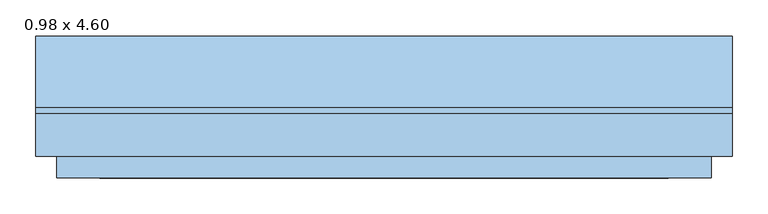
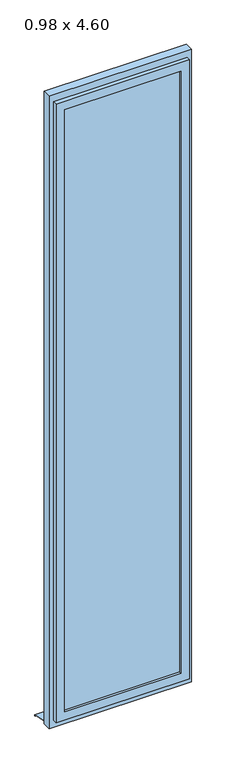
"""IFC4 building model written with IfcOpenShell, lengths in millimetres: window geometry, Fenstertür 1-flg : 0.98 x 4.60."""

from ifc_helpers import new_model, si_unit, frame, origin, place, context, project, spatial, polyline, outline, extrude, faceted_brep, source, transform, mapped, element, save


def window_0_98_x_4_60_477bf46f(model_context):
    return source(origin(), model_context, "Body", "SolidModel", [
        extrude(outline(polyline([(4600.0, 490.0), (4600.0, -490.0), (0.0, -490.0), (0.0, 490.0), (4600.0, 490.0)]), holes=[polyline([(4520.0, 430.0), (80.0, 430.0), (80.0, -430.0), (4520.0, -430.0), (4520.0, 430.0)])]), frame((0.0, -80.0, 0.0), z_axis=(0.0, 1.0, 0.0), x_axis=(0.0, 0.0, 1.0)), (0.0, 0.0, 1.0), 60.0),
        faceted_brep([(460.0, -80.0, 4550.0), (460.0, -110.0, 4550.0), (460.0, -110.0, 50.0), (460.0, -80.0, 50.0), (-460.0, -110.0, 4550.0), (-460.0, -110.0, 50.0), (400.0, -110.0, 110.0), (-400.0, -110.0, 110.0), (-400.0, -110.0, 4490.0), (400.0, -110.0, 4490.0), (-460.0, -80.0, 50.0), (-460.0, -80.0, 4550.0), (430.0, -80.0, 4520.0), (-430.0, -80.0, 4520.0), (-430.0, -80.0, 80.0), (430.0, -80.0, 80.0), (430.0, -50.0, 4520.0), (430.0, -50.0, 80.0), (-430.0, -50.0, 80.0), (-430.0, -50.0, 4520.0), (400.0, -50.0, 4490.0), (-400.0, -50.0, 4490.0), (-400.0, -50.0, 110.0), (400.0, -50.0, 110.0)], [[[0, 1, 2, 3]], [[1, 4, 5, 2], [6, 7, 8, 9]], [[3, 2, 5, 10]], [[3, 10, 11, 0], [12, 13, 14, 15]], [[16, 12, 15, 17]], [[17, 15, 14, 18]], [[17, 18, 19, 16], [20, 21, 22, 23]], [[9, 20, 23, 6]], [[6, 23, 22, 7]], [[10, 5, 4, 11]], [[18, 14, 13, 19]], [[7, 22, 21, 8]], [[11, 4, 1, 0]], [[19, 13, 12, 16]], [[8, 21, 20, 9]]]),
        extrude(outline(polyline([(-9.9778457, 20.0), (90.0, 0.0), (90.0, -10.0), (88.0, -10.0), (88.0, -1.6395366), (-10.1759277, 18.0), (-20.0, 18.0), (-20.0, 20.0), (-9.9778457, 20.0)])), frame((-490.0, 0.0, 0.0), z_axis=(1.0, 0.0, 0.0), x_axis=(0.0, 1.0, 0.0)), (0.0, 0.0, 1.0), 980.0),
        extrude(outline(polyline([(400.0, -95.0), (-400.0, -95.0), (-400.0, -65.0), (400.0, -65.0), (400.0, -95.0)])), frame((0.0, 0.0, 110.0), z_axis=(0.0, 0.0, 1.0), x_axis=(1.0, 0.0, 0.0)), (0.0, 0.0, 1.0), 4380.0),
    ])


if __name__ == "__main__":
    model = new_model("IFC4")
    model_context = context("Model", 3, world=origin())
    ifc_project = project(units=[si_unit("LENGTHUNIT", "METRE", prefix="MILLI")], contexts=[model_context])
    site = spatial("IfcSite", under=ifc_project)
    building = spatial("IfcBuilding", under=site)
    placement = place(None, origin())
    window_0_98_x_4_60_shape = window_0_98_x_4_60_477bf46f(model_context)
    element("IfcWindow", 1, ObjectType="Fenstertür 1-flg : 0.98 x 4.60", at=placement, inside=building, context=model_context, shape_type="MappedRepresentation", body=[
        mapped(window_0_98_x_4_60_shape, transform((0.0, 0.0, 0.0), x_axis=(1.0, 0.0, 0.0), y_axis=(0.0, 1.0, 0.0), z_axis=(0.0, 0.0, 1.0))),
    ])
    save(model, "model.ifc")

# Revit data of these elements
# Type "Fenstertür 1-flg : 0.98 x 4.60"
#   Type Mark = "61"
#   Operation = "SinglePanel"
#   Construction Type Id = "SGL"
#   Keynote = "16.05.01"
#   Analytic Construction = "Große Fenster mit Einfachverglasung"
#   Visual Light Transmittance = 0.9
#   Solar Heat Gain Coefficient = 0.86
#   Rough Width = 0.980 m
#   Rough Height = 4.600 m
#   Heat Transfer Coefficient (U) = 5.5617 W/(m²·K)
#   Rahmentiefe = 0.060 m
#   Rahmenhöhe unten = 0.080 m
#   Höhe oberer  Rahmen = 0.080 m
#   Rahmenbreite = 0.060 m
#   Height = 4.600 m
#   Tiefe Flügel = 0.060 m
#   Flügelbreite = 0.060 m
#   Einbautiefe (von außen) [instance default] = 0.080 m
#   Width = 0.980 m
#   Sichtbarkeit Sturzlinien [instance default] = yes
#   Öffnungsrichtung oben [instance default] = yes
#   Öffnungsrichtung in Draufsicht anzeigen [instance default] = yes
#   Drehflügel 1 [instance default] = yes
#   Bild [instance default] = none
#   Glas [instance default] = none
#   Fensterflügel [instance default] = none
#   Äußere Fensterbank [instance default] = none
#   Wall Closure = (empty or 0)
# Element 1 (IfcWindow, "Fenstertür 1-flg : 0.98 x 4.60")
#   Materials on its faces: "Kunststoff - Weiß", "Glas"
# Materials
#   "Kunststoff - Weiß": class "Kunststoff", colour RGB 249 249 249, transparency 0, Cost = 0
#   "Glas": class "Glas", colour RGB 0 0 255, transparency 0.75, Comments = "Render-Darstellung nicht aktualisiert ", Cost = 0
